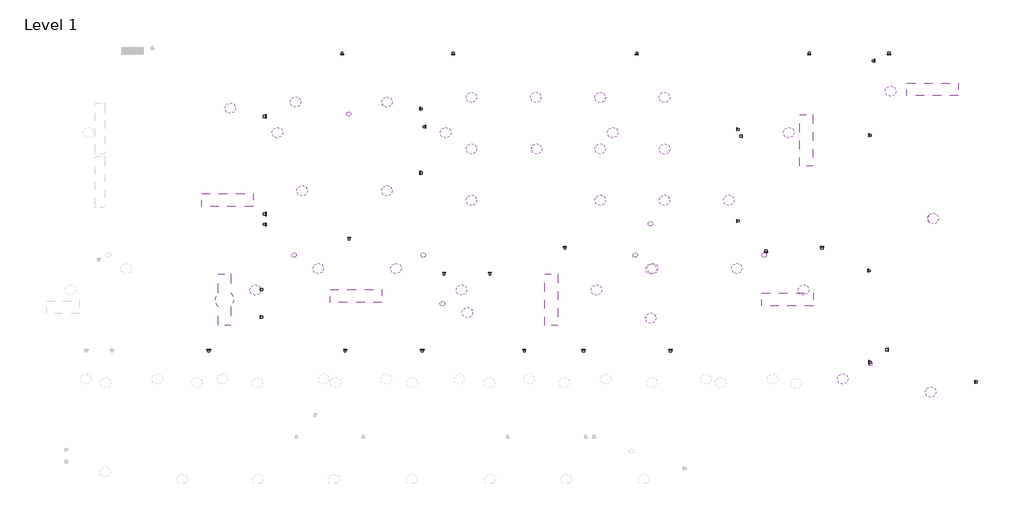
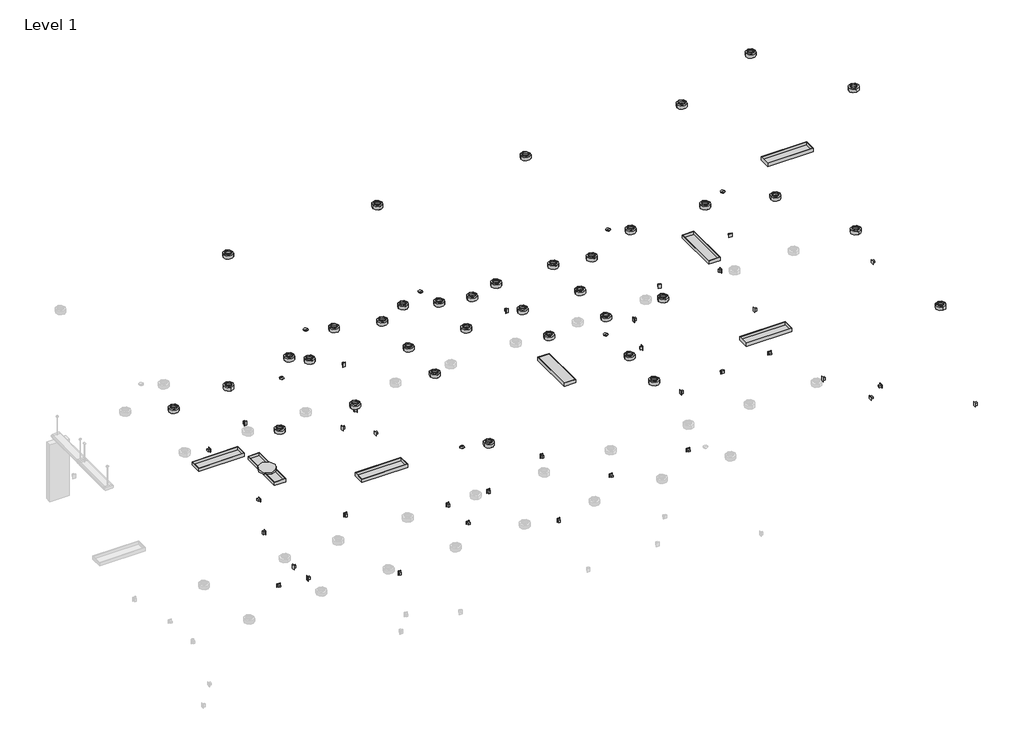
# One storey, part 3 of 3: 43 light fixtures, 22 proxies, 20 switching devices.
# Revit data of these elements (continued)
# Element 74 (IfcSwitchingDevice, "Lighting Switches One Way : One Way Switch") (continued)
#   Mark = "33"
#   COBie.CreatedBy = "info@mma.ie"
#   COBie.CreatedOn = "2017-07-25T10:15:16"
#   COBie.Component.Name = "Lighting Switches One Way_33"
#   COBie.Component.Space = "113"
#   COBie.Component.Description = "Lighting Switches One Way: One Way Switch"
#   Notes = "n/a"
#   Floor Level = "Level 1"
#   COBie = yes
#   Phase Created = New Construction
# Element 75 (IfcSwitchingDevice, "Lighting Switches One Way : One Way Switch")
#   Comments = "Switch"
#   Mark = "34"
#   COBie.CreatedBy = "info@mma.ie"
#   COBie.CreatedOn = "2017-07-25T10:15:16"
#   COBie.Component.Name = "Lighting Switches One Way_34"
#   COBie.Component.Space = "112"
#   COBie.Component.Description = "Lighting Switches One Way: One Way Switch"
#   Notes = "n/a"
#   Floor Level = "Level 1"
#   COBie = yes
#   Phase Created = New Construction
# Element 76 (IfcSwitchingDevice, "Lighting Switches One Way : One Way Switch")
#   Comments = "Switch"
#   Mark = "35"
#   COBie.CreatedBy = "info@mma.ie"
#   COBie.CreatedOn = "2017-07-25T10:15:16"
#   COBie.Component.Name = "Lighting Switches One Way_35"
#   COBie.Component.Space = "111"
#   COBie.Component.Description = "Lighting Switches One Way: One Way Switch"
#   Notes = "n/a"
#   Floor Level = "Level 1"
#   COBie = yes
#   Phase Created = New Construction
# Element 77 (IfcSwitchingDevice, "Lighting Switches One Way : One Way Switch")
#   Comments = "Switch"
#   Mark = "36"
#   COBie.CreatedBy = "info@mma.ie"
#   COBie.CreatedOn = "2017-07-25T10:15:16"
#   COBie.Component.Name = "Lighting Switches One Way_36"
#   COBie.Component.Space = "115"
#   COBie.Component.Description = "Lighting Switches One Way: One Way Switch"
#   Notes = "n/a"
#   Floor Level = "Level 1"
#   COBie = yes
#   Phase Created = New Construction
# Element 78 (IfcSwitchingDevice, "Lighting Switches One Way : One Way Switch")
#   Comments = "Switch"
#   Mark = "37"
#   COBie.CreatedBy = "info@mma.ie"
#   COBie.CreatedOn = "2017-07-25T10:15:16"
#   COBie.Component.Name = "Lighting Switches One Way_37"
#   COBie.Component.Space = "110"
#   COBie.Component.Description = "Lighting Switches One Way: One Way Switch"
#   Notes = "n/a"
#   Floor Level = "Level 1"
#   COBie = yes
#   Phase Created = New Construction
# Element 79 (IfcSwitchingDevice, "Lighting Switches One Way : One Way Switch")
#   Comments = "Switch"
#   Mark = "38"
#   COBie.CreatedBy = "info@mma.ie"
#   COBie.CreatedOn = "2017-07-25T10:15:16"
#   COBie.Component.Name = "Lighting Switches One Way_38"
#   COBie.Component.Space = "109"
#   COBie.Component.Description = "Lighting Switches One Way: One Way Switch"
#   Notes = "n/a"
#   Floor Level = "Level 1"
#   COBie = yes
#   Phase Created = New Construction
# Element 80 (IfcSwitchingDevice, "Lighting Switches One Way : One Way Switch")
#   Comments = "Switch"
#   Mark = "39"
#   COBie.ExternalIdentifier = ""
#   COBie.CreatedBy = "info@mma.ie"
#   COBie.CreatedOn = "2017-07-25T10:15:16"
#   COBie.Component.Name = "Lighting Switches One Way_39"
#   COBie.Component.Space = "108"
#   COBie.Component.Description = "Lighting Switches One Way: One Way Switch"
#   Notes = "n/a"
#   Floor Level = "Level 1"
#   COBie = yes
#   Phase Created = New Construction
# Element 81 (IfcSwitchingDevice, "Lighting Switches One Way : One Way Switch")
#   Comments = "Switch"
#   Mark = "40"
#   COBie.CreatedBy = "info@mma.ie"
#   COBie.CreatedOn = "2017-07-25T10:15:16"
#   COBie.Component.Name = "Lighting Switches One Way_40"
#   COBie.Component.Space = "108"
#   COBie.Component.Description = "Lighting Switches One Way: One Way Switch"
#   Notes = "n/a"
#   Floor Level = "Level 1"
#   COBie = yes
#   Phase Created = New Construction
# Element 82 (IfcSwitchingDevice, "Lighting Switches One Way : One Way Switch")
#   Comments = "Switch"
#   Mark = "41"
#   COBie.CreatedBy = "info@mma.ie"
#   COBie.CreatedOn = "2017-07-25T10:15:16"
#   COBie.Component.Name = "Lighting Switches One Way_41"
#   COBie.Component.Space = "108"
#   COBie.Component.Description = "Lighting Switches One Way: One Way Switch"
#   Notes = "n/a"
#   Floor Level = "Level 1"
#   COBie = yes
#   Phase Created = New Construction
# Element 83 (IfcSwitchingDevice, "Lighting Switches Two Way : Two Way Switch")
#   Comments = "Switch"
#   Mark = "1"
#   COBie.CreatedBy = "info@mma.ie"
#   COBie.CreatedOn = "2017-07-25T10:15:16"
#   COBie.Component.Name = "Lighting Switches Two Way_1"
#   COBie.Component.Space = "117"
#   COBie.Component.Description = "Lighting Switches Two Way: Two Way Switch"
#   Notes = "n/a"
#   Floor Level = "Level 1"
#   COBie = yes
#   Phase Created = New Construction
# Element 84 (IfcSwitchingDevice, "Lighting Switches Two Way : Two Way Switch")
#   Comments = "Switch"
#   Mark = "4"
#   COBie.CreatedBy = "info@mma.ie"
#   COBie.CreatedOn = "2017-07-25T10:15:16"
#   COBie.Component.Name = "Lighting Switches Two Way_4"
#   COBie.Component.Space = "217"
#   COBie.Component.Description = "Lighting Switches Two Way: Two Way Switch"
#   Notes = "n/a"
#   Floor Level = "Level 2"
#   COBie = yes
#   Phase Created = New Construction
# Element 85 (IfcSwitchingDevice, "Lighting Switches Two Way : Two Way Switch")
#   Comments = "Switch"
#   Mark = "2"
#   COBie.CreatedBy = "info@mma.ie"
#   COBie.CreatedOn = "2017-07-25T10:15:16"
#   COBie.Component.Name = "Lighting Switches Two Way_2"
#   COBie.Component.Space = "116"
#   COBie.Component.Description = "Lighting Switches Two Way: Two Way Switch"
#   Notes = "n/a"
#   Floor Level = "Level 1"
#   COBie = yes
#   Phase Created = New Construction
# Materials
#   "Stainless Steel": class "Metal", colour RGB 120 120 120, transparency 0, Description = "Stainless Steel 18/8", Cost = 0
#   "Phase - Demo": class "System", colour RGB 255 0 0, transparency 0.4
#   "Metal - Paint Finish - Ivory, Glossy": class "Paint", colour RGB 247 247 239, transparency 0, Comments = "Rendering appearance not upgraded "
#   "Glass - White, High Luminance": class "Glass", colour RGB 249 250 249, transparency 0.8
#   "Metal - Paint Finish - Dark Grey, Matt": class "Paint", colour RGB 98 98 98, transparency 0
#   "Phase-Demo": class "Unassigned", colour RGB 0 0 0, transparency 0.4, Cost = 0
#   "Plastic-White-Gloss": class "Plastic", colour RGB 255 255 255, transparency 0, Cost = 0
#   "Metal - Chrome": class "Metal", colour RGB 17 17 17, transparency 0, Comments = "Rendering appearance not upgraded "
# Space at (2185.935, -3546.129) mm, phase "New Construction", upper level "Level 1", upper offset 2000 mm, lower offset 0 mm
#   Number = "128"
#   Name = "External Space Level 1"
#   Classification.Space.Number = "13-25 17"
#   Classification.Space.Description = "External Circulation Spaces"
#   COBie.CreatedBy = "info@mma.ie"
#   COBie.CreatedOn = "2017-07-25T10:15:16"
#   COBie.Space.Name = "128"
#   COBie.Space.Category = "13-25 17 : External Circulation Spaces"
#   COBie.Space.Description = "External Circulation Spaces"
#   Actual Lighting Load per area = 0
#   Actual Power Load per area = 0
#   Sensible Heat Gain per person = 0
#   Specified Lighting Load = 0
#   Specified Power Load = 0
#   Latent Heat Gain per person = 0
#   Total Heat Gain per person = 0
#   Area per Person = 0
#   Number of People = 24.3597 (stored number, unit not read)
#   COBie.Space.UsableHeight = 2000 mm
#   COBie.Space.GrossArea = 695.992 m²
#   COBie.Space.NetArea = 0 m²
#   Lighting Load Units = 0
#   Power Load Units = 0
#   Return Airflow = 0
#   Occupancy Unit = -1
#   Condition Type = 2
#   COBie = yes
#   Construction Type = none
# Space at (25106.449, 9340.039) mm, phase "New Construction", upper level "Level 2", upper offset -200 mm, lower offset 0 mm
#   Number = "111"
#   Name = "Storage"
#   Classification.Space.Number = "13-63 13 11"
#   Classification.Space.Description = "Storage Room"
#   COBie.CreatedBy = "info@mma.ie"
#   COBie.CreatedOn = "2017-07-25T10:15:16"
#   COBie.Space.Name = "111"
#   COBie.Space.Category = "13-63 13 11 : Storage Room"
#   COBie.Space.Description = "Storage"
#   Actual Lighting Load per area = 0
#   Actual Power Load per area = 0
#   Sensible Heat Gain per person = 0
#   Specified Lighting Load = 0
#   Specified Power Load = 0
#   Latent Heat Gain per person = 0
#   Total Heat Gain per person = 0
#   Area per Person = 0
#   Number of People = 9.98655 (stored number, unit not read)
#   COBie.Space.UsableHeight = 3600 mm
#   COBie.Space.GrossArea = 5.21302 m²
#   COBie.Space.NetArea = 0 m²
#   Lighting Load Units = 0
#   Power Load Units = 0
#   Return Airflow = 0
#   Occupancy Unit = -1
#   Condition Type = 2
#   COBie = yes
#   Construction Type = none
# Space at (4303.158, 2552.548) mm, phase "New Construction", upper level "Level 2", upper offset -200 mm, lower offset 0 mm
#   Number = "124"
#   Name = "Closet"
#   Classification.Space.Number = "13-63 13 13"
#   Classification.Space.Description = "Closet"
#   COBie.CreatedBy = "info@mma.ie"
#   COBie.CreatedOn = "2017-07-25T10:15:16"
#   COBie.Space.Name = "124"
#   COBie.Space.Category = "13-63 13 13 : Closet"
#   COBie.Space.Description = "Closet"
#   Actual Lighting Load per area = 0
#   Actual Power Load per area = 0
#   Sensible Heat Gain per person = 0
#   Specified Lighting Load = 0
#   Specified Power Load = 0
#   Latent Heat Gain per person = 0
#   Total Heat Gain per person = 0
#   Area per Person = 0
#   Number of People = 5.16564 (stored number, unit not read)
#   COBie.Space.UsableHeight = 3600 mm
#   COBie.Space.GrossArea = 1.97733 m²
#   COBie.Space.NetArea = 0 m²
#   Lighting Load Units = 0
#   Power Load Units = 0
#   Return Airflow = 0
#   Occupancy Unit = -1
#   Condition Type = 2
#   COBie = yes
#   Construction Type = none
# Space at (-3347.4, 10795.629) mm, phase "New Construction", upper level "Level 2", upper offset 0 mm, lower offset 0 mm
#   Number = "001"
#   Name = "Exercise Terrace"
#   Classification.Space.Number = "13-33 11 15 41"
#   Classification.Space.Description = "Exercise Space"
#   COBie.CreatedBy = "info@mma.ie"
#   COBie.CreatedOn = "2017-07-25T10:15:16"
#   COBie.Space.Name = "001"
#   COBie.Space.Category = "13-33 11 15 41 : Exercise Space"
#   COBie.Space.Description = "Exercise Terrace"
#   Actual Lighting Load per area = 0
#   Actual Power Load per area = 0
#   Sensible Heat Gain per person = 0
#   Specified Lighting Load = 0
#   Specified Power Load = 0
#   Latent Heat Gain per person = 0
#   Total Heat Gain per person = 0
#   Area per Person = 0
#   Number of People = 1.64607 (stored number, unit not read)
#   COBie.Space.UsableHeight = 3800 mm
#   COBie.Space.GrossArea = 47.0306 m²
#   COBie.Space.NetArea = 0 m²
#   Lighting Load Units = 0
#   Power Load Units = 0
#   Return Airflow = 0
#   Occupancy Unit = -1
#   Condition Type = 2
#   COBie = yes
#   Construction Type = none
# Space at (19013.47, -3392.114) mm, phase "New Construction", upper level "Level 2", upper offset 0 mm, lower offset 0 mm
#   Number = "002"
#   Name = "Terrace"
#   Classification.Space.Number = "13-33 15 19"
#   Classification.Space.Description = "Recreational Deck"
#   COBie.CreatedBy = "info@mma.ie"
#   COBie.CreatedOn = "2017-07-25T10:15:16"
#   COBie.Space.Name = "002"
#   COBie.Space.Category = "13-33 15 19 : Recreational Deck"
#   COBie.Space.Description = "Terrace"
#   Actual Lighting Load per area = 0
#   Actual Power Load per area = 0
#   Sensible Heat Gain per person = 0
#   Specified Lighting Load = 0
#   Specified Power Load = 0
#   Latent Heat Gain per person = 0
#   Total Heat Gain per person = 0
#   Area per Person = 0
#   Number of People = 4.71044 (stored number, unit not read)
#   COBie.Space.UsableHeight = 3800 mm
#   COBie.Space.GrossArea = 134.584 m²
#   COBie.Space.NetArea = 0 m²
#   Lighting Load Units = 0
#   Power Load Units = 0
#   Return Airflow = 0
#   Occupancy Unit = -1
#   Condition Type = 2
#   COBie = yes
#   Construction Type = none
# Space at (33637.505, 9582.548) mm, phase "New Construction", upper level "Level 2", upper offset 0 mm, lower offset 0 mm
#   Number = "116"
#   Name = "Stair 2"
#   Classification.Space.Number = "13-23 11 13"
#   Classification.Space.Description = "Stairway"
#   COBie.CreatedBy = "info@mma.ie"
#   COBie.CreatedOn = "2017-07-25T10:15:16"
#   COBie.Space.Name = "116"
#   COBie.Space.Category = "13-23 11 13 : Stairway"
#   COBie.Space.Description = "Stair 2"
#   Actual Lighting Load per area = 0
#   Actual Power Load per area = 0
#   Sensible Heat Gain per person = 0
#   Specified Lighting Load = 0
#   Specified Power Load = 0
#   Latent Heat Gain per person = 0
#   Total Heat Gain per person = 0
#   Area per Person = 0
#   Number of People = 0.462 (stored number, unit not read)
#   COBie.Space.UsableHeight = 3800 mm
#   COBie.Space.GrossArea = 11.862 m²
#   COBie.Space.NetArea = 0 m²
#   Lighting Load Units = 0
#   Power Load Units = 0
#   Return Airflow = 0
#   Occupancy Unit = -1
#   Condition Type = 2
#   COBie = yes
#   Construction Type = none
# Space at (13307.53, 9198.989) mm, phase "New Construction", upper level "Level 2", upper offset -200 mm, lower offset 0 mm
#   Number = "104"
#   Name = "Storage"
#   Classification.Space.Number = "13-63 13 11"
#   Classification.Space.Description = "Storage Room"
#   COBie.CreatedBy = "info@mma.ie"
#   COBie.CreatedOn = "2017-07-25T10:15:16"
#   COBie.Space.Name = "104"
#   COBie.Space.Category = "13-63 13 11 : Storage Room"
#   COBie.Space.Description = "Storage"
#   Actual Lighting Load per area = 0
#   Actual Power Load per area = 0
#   Sensible Heat Gain per person = 0
#   Specified Lighting Load = 0
#   Specified Power Load = 0
#   Latent Heat Gain per person = 0
#   Total Heat Gain per person = 0
#   Area per Person = 0
#   Number of People = 0.36309 (stored number, unit not read)
#   COBie.Space.UsableHeight = 3600 mm
#   COBie.Space.GrossArea = 10.374 m²
#   COBie.Space.NetArea = 0 m²
#   Lighting Load Units = 0
#   Power Load Units = 0
#   Return Airflow = 0
#   Occupancy Unit = -1
#   Condition Type = 2
#   COBie = yes
#   Construction Type = none
# Space at (17223.661, 11648.121) mm, phase "New Construction", upper level "Level 2", upper offset -200 mm, lower offset 0 mm
#   Number = "107"
#   Name = "Closet"
#   Classification.Space.Number = "13-63 13 13"
#   Classification.Space.Description = "Closet"
#   COBie.CreatedBy = "info@mma.ie"
#   COBie.CreatedOn = "2017-07-25T10:15:16"
#   COBie.Space.Name = "107"
#   COBie.Space.Category = "13-63 13 13 : Closet"
#   COBie.Space.Description = "Closet"
#   Actual Lighting Load per area = 0
#   Actual Power Load per area = 0
#   Sensible Heat Gain per person = 0
#   Specified Lighting Load = 0
#   Specified Power Load = 0
#   Latent Heat Gain per person = 0
#   Total Heat Gain per person = 0
#   Area per Person = 0
#   Number of People = 0.0932222 (stored number, unit not read)
#   COBie.Space.UsableHeight = 3600 mm
#   COBie.Space.GrossArea = 2.66349 m²
#   COBie.Space.NetArea = 0 m²
#   Lighting Load Units = 0
#   Power Load Units = 0
#   Return Airflow = 0
#   Occupancy Unit = -1
#   Condition Type = 2
#   COBie = yes
#   Construction Type = none
# Space at (17223.661, 9449.227) mm, phase "New Construction", upper level "Level 2", upper offset -200 mm, lower offset 0 mm
#   Number = "109"
#   Name = "Elec/Tel"
#   Classification.Space.Number = "13-23 19 27"
#   Classification.Space.Description = "Electrical Room"
#   COBie.CreatedBy = "info@mma.ie"
#   COBie.CreatedOn = "2017-07-25T10:15:16"
#   COBie.Space.Name = "109"
#   COBie.Space.Category = "13-23 19 27 : Electrical Room"
#   COBie.Space.Description = "Elec/Tel"
#   Actual Lighting Load per area = 0
#   Actual Power Load per area = 0
#   Sensible Heat Gain per person = 0
#   Specified Lighting Load = 0
#   Specified Power Load = 0
#   Latent Heat Gain per person = 0
#   Total Heat Gain per person = 0
#   Area per Person = 0
#   Number of People = 0.141204 (stored number, unit not read)
#   COBie.Space.UsableHeight = 3600 mm
#   COBie.Space.GrossArea = 4.03441 m²
#   COBie.Space.NetArea = 0 m²
#   Lighting Load Units = 0
#   Power Load Units = 0
#   Return Airflow = 0
#   Occupancy Unit = -1
#   Condition Type = 2
#   COBie = yes
#   Construction Type = none
# Space at (20994.03, 9449.227) mm, phase "New Construction", upper level "Level 2", upper offset -200 mm, lower offset 0 mm
#   Number = "110"
#   Name = "Laundry"
#   Classification.Space.Number = "13-65 17"
#   Classification.Space.Description = "Laundry Room"
#   COBie.CreatedBy = "info@mma.ie"
#   COBie.CreatedOn = "2017-07-25T10:15:16"
#   COBie.Space.Name = "110"
#   COBie.Space.Category = "13-65 17 : Laundry Room"
#   COBie.Space.Description = "Laundry"
#   Actual Lighting Load per area = 0
#   Actual Power Load per area = 0
#   Sensible Heat Gain per person = 0
#   Specified Lighting Load = 0
#   Specified Power Load = 0
#   Latent Heat Gain per person = 0
#   Total Heat Gain per person = 0
#   Area per Person = 0
#   Number of People = 0.437432 (stored number, unit not read)
#   COBie.Space.UsableHeight = 3600 mm
#   COBie.Space.GrossArea = 12.4981 m²
#   COBie.Space.NetArea = 0 m²
#   Lighting Load Units = 0
#   Power Load Units = 0
#   Return Airflow = 0
#   Occupancy Unit = -1
#   Condition Type = 2
#   COBie = yes
#   Construction Type = none
# Space at (9483.268, 9198.989) mm, phase "New Construction", upper level "Level 2", upper offset -200 mm, lower offset 0 mm
#   Number = "103"
#   Name = "Toilet"
#   Classification.Space.Number = "13-65 13 13"
#   Classification.Space.Description = "Toilet Space"
#   COBie.CreatedBy = "info@mma.ie"
#   COBie.CreatedOn = "2017-07-25T10:15:16"
#   COBie.Space.Name = "103"
#   COBie.Space.Category = "13-65 13 13 : Toilet Space"
#   COBie.Space.Description = "Toilet"
#   Actual Lighting Load per area = 0
#   Actual Power Load per area = 0
#   Sensible Heat Gain per person = 0
#   Specified Lighting Load = 0
#   Specified Power Load = 0
#   Latent Heat Gain per person = 0
#   Total Heat Gain per person = 0
#   Area per Person = 0
#   Number of People = 0.146893 (stored number, unit not read)
#   COBie.Space.UsableHeight = 3600 mm
#   COBie.Space.GrossArea = 4.19694 m²
#   COBie.Space.NetArea = 0 m²
#   Lighting Load Units = 0
#   Power Load Units = 0
#   Return Airflow = 0
#   Occupancy Unit = -1
#   Condition Type = 2
#   COBie = yes
#   Construction Type = none
# Space at (7140.705, 9198.989) mm, phase "New Construction", upper level "Level 2", upper offset -200 mm, lower offset 0 mm
#   Number = "102"
#   Name = "Toilet"
#   Classification.Space.Number = "13-65 13 13"
#   Classification.Space.Description = "Toilet Space"
#   COBie.CreatedBy = "info@mma.ie"
#   COBie.CreatedOn = "2017-07-25T10:15:16"
#   COBie.Space.Name = "102"
#   COBie.Space.Category = "13-65 13 13 : Toilet Space"
#   COBie.Space.Description = "Toilet"
#   Actual Lighting Load per area = 0
#   Actual Power Load per area = 0
#   Sensible Heat Gain per person = 0
#   Specified Lighting Load = 0
#   Specified Power Load = 0
#   Latent Heat Gain per person = 0
#   Total Heat Gain per person = 0
#   Area per Person = 0
#   Number of People = 0.146751 (stored number, unit not read)
#   COBie.Space.UsableHeight = 3600 mm
#   COBie.Space.GrossArea = 4.19289 m²
#   COBie.Space.NetArea = 0 m²
#   Lighting Load Units = 0
#   Power Load Units = 0
#   Return Airflow = 0
#   Occupancy Unit = -1
#   Condition Type = 2
#   COBie = yes
#   Construction Type = none
# Space at (17223.661, 13855.183) mm, phase "New Construction", upper level "Level 2", upper offset -200 mm, lower offset 0 mm
#   Number = "106"
#   Name = "Bath"
#   Classification.Space.Number = "13-65 13"
#   Classification.Space.Description = "Bathroom"
#   COBie.CreatedBy = "info@mma.ie"
#   COBie.CreatedOn = "2017-07-25T10:15:16"
#   COBie.Space.Name = "106"
#   COBie.Space.Category = "13-65 13 : Bathroom"
#   COBie.Space.Description = "Bath"
#   Actual Lighting Load per area = 0
#   Actual Power Load per area = 0
#   Sensible Heat Gain per person = 0
#   Specified Lighting Load = 0
#   Specified Power Load = 0
#   Latent Heat Gain per person = 0
#   Total Heat Gain per person = 0
#   Area per Person = 0
#   Number of People = 0.141421 (stored number, unit not read)
#   COBie.Space.UsableHeight = 3600 mm
#   COBie.Space.GrossArea = 4.0406 m²
#   COBie.Space.NetArea = 0 m²
#   Lighting Load Units = 0
#   Power Load Units = 0
#   Return Airflow = 0
#   Occupancy Unit = -1
#   Condition Type = 2
#   COBie = yes
#   Construction Type = none
# Space at (19950.249, 12967.977) mm, phase "New Construction", upper level "Level 2", upper offset -200 mm, lower offset 0 mm
#   Number = "108"
#   Name = "Break Room"
#   Classification.Space.Number = "13-57 17 13"
#   Classification.Space.Description = "Break Room"
#   COBie.CreatedBy = "info@mma.ie"
#   COBie.CreatedOn = "2017-07-25T10:15:16"
#   COBie.Space.Name = "108"
#   COBie.Space.Category = "13-57 17 13 : Break Room"
#   COBie.Space.Description = "Break Room"
#   Actual Lighting Load per area = 0
#   Actual Power Load per area = 0
#   Sensible Heat Gain per person = 0
#   Specified Lighting Load = 0
#   Specified Power Load = 0
#   Latent Heat Gain per person = 0
#   Total Heat Gain per person = 0
#   Area per Person = 0
#   Number of People = 0.538984 (stored number, unit not read)
#   COBie.Space.UsableHeight = 3600 mm
#   COBie.Space.GrossArea = 15.3995 m²
#   COBie.Space.NetArea = 0 m²
#   Lighting Load Units = 0
#   Power Load Units = 0
#   Return Airflow = 0
#   Occupancy Unit = -1
#   Condition Type = 2
#   COBie = yes
#   Construction Type = none
# Space at (33531.255, 14017.548) mm, phase "New Construction", upper level "Level 2", upper offset -200 mm, lower offset 0 mm
#   Number = "115"
#   Name = "Outdoor Storage"
#   Classification.Space.Number = "13-63 13 11"
#   Classification.Space.Description = "Storage Room"
#   COBie.CreatedBy = "info@mma.ie"
#   COBie.CreatedOn = "2017-07-25T10:15:16"
#   COBie.Space.Name = "115"
#   COBie.Space.Category = "13-63 13 11 : Storage Room"
#   COBie.Space.Description = "Outdoor Storage"
#   Actual Lighting Load per area = 0
#   Actual Power Load per area = 0
#   Sensible Heat Gain per person = 0
#   Specified Lighting Load = 0
#   Specified Power Load = 0
#   Latent Heat Gain per person = 0
#   Total Heat Gain per person = 0
#   Area per Person = 0
#   Number of People = 0.183416 (stored number, unit not read)
#   COBie.Space.UsableHeight = 3600 mm
#   COBie.Space.GrossArea = 5.24046 m²
#   COBie.Space.NetArea = 0 m²
#   Lighting Load Units = 0
#   Power Load Units = 0
#   Return Airflow = 0
#   Occupancy Unit = -1
#   Condition Type = 2
#   COBie = yes
#   Construction Type = none
# Space at (12208.83, 12750.239) mm, phase "New Construction", upper level "Level 2", upper offset -200 mm, lower offset 0 mm
#   Number = "105"
#   Name = "Mechanical Room"
#   Classification.Space.Number = "13-23 19"
#   Classification.Space.Description = "Utility Equipment Room"
#   COBie.CreatedBy = "info@mma.ie"
#   COBie.CreatedOn = "2017-07-25T10:15:16"
#   COBie.Space.Name = "105"
#   COBie.Space.Category = "13-23 19 : Utility Equipment Room"
#   COBie.Space.Description = "Mechanical Room"
#   Actual Lighting Load per area = 0
#   Actual Power Load per area = 0
#   Sensible Heat Gain per person = 0
#   Specified Lighting Load = 0
#   Specified Power Load = 0
#   Latent Heat Gain per person = 0
#   Total Heat Gain per person = 0
#   Area per Person = 0
#   Number of People = 1.28766 (stored number, unit not read)
#   COBie.Space.UsableHeight = 3600 mm
#   COBie.Space.GrossArea = 36.7902 m²
#   COBie.Space.NetArea = 0 m²
#   Lighting Load Units = 0
#   Power Load Units = 0
#   Return Airflow = 0
#   Occupancy Unit = -1
#   Condition Type = 2
#   COBie = yes
#   Construction Type = none
# Space at (10643.485, 2189.772) mm, phase "New Construction", upper level "Level 2", upper offset -200 mm, lower offset 0 mm
#   Number = "121"
#   Name = "Living Room"
#   Classification.Space.Number = "13-65"
#   Classification.Space.Description = "Private Residential Spaces"
#   COBie.CreatedBy = "info@mma.ie"
#   COBie.CreatedOn = "2017-07-25T10:15:16"
#   COBie.Space.Name = "121"
#   COBie.Space.Category = "13-57 17 11 : Rest Area"
#   COBie.Space.Description = "Living Room"
#   Actual Lighting Load per area = 0
#   Actual Power Load per area = 0
#   Sensible Heat Gain per person = 0
#   Specified Lighting Load = 0
#   Specified Power Load = 0
#   Latent Heat Gain per person = 0
#   Total Heat Gain per person = 0
#   Area per Person = 0
#   Number of People = 0.615682 (stored number, unit not read)
#   COBie.Space.UsableHeight = 3600 mm
#   COBie.Space.GrossArea = 17.5909 m²
#   COBie.Space.NetArea = 0 m²
#   Lighting Load Units = 0
#   Power Load Units = 0
#   Return Airflow = 0
#   Occupancy Unit = -1
#   Condition Type = 2
#   COBie = yes
#   Construction Type = none
# Space at (9068.854, 5264.772) mm, phase "New Construction", upper level "Level 2", upper offset -200 mm, lower offset 0 mm
#   Number = "122"
#   Name = "Closet"
#   Classification.Space.Number = "13-63 13 13"
#   Classification.Space.Description = "Closet"
#   COBie.CreatedBy = "info@mma.ie"
#   COBie.CreatedOn = "2017-07-25T10:15:16"
#   COBie.Space.Name = "122"
#   COBie.Space.Category = "13-63 13 13 : Closet"
#   COBie.Space.Description = "Closet"
#   Actual Lighting Load per area = 0
#   Actual Power Load per area = 0
#   Sensible Heat Gain per person = 0
#   Specified Lighting Load = 0
#   Specified Power Load = 0
#   Latent Heat Gain per person = 0
#   Total Heat Gain per person = 0
#   Area per Person = 0
#   Number of People = 0.113917 (stored number, unit not read)
#   COBie.Space.UsableHeight = 3600 mm
#   COBie.Space.GrossArea = 3.25478 m²
#   COBie.Space.NetArea = 0 m²
#   Lighting Load Units = 0
#   Power Load Units = 0
#   Return Airflow = 0
#   Occupancy Unit = -1
#   Condition Type = 2
#   COBie = yes
#   Construction Type = none
# Space at (3785.935, 3859.219) mm, phase "New Construction", upper level "Level 2", upper offset 0 mm, lower offset 0 mm
#   Number = "125"
#   Name = "Stair 1"
#   Classification.Space.Number = "13-23 11 13"
#   Classification.Space.Description = "Stairway"
#   COBie.CreatedBy = "info@mma.ie"
#   COBie.CreatedOn = "2017-07-25T10:15:16"
#   COBie.Space.Name = "125"
#   COBie.Space.Category = "13-23 11 13 : Stairway"
#   COBie.Space.Description = "Stair 1"
#   Actual Lighting Load per area = 0
#   Actual Power Load per area = 0
#   Sensible Heat Gain per person = 0
#   Specified Lighting Load = 0
#   Specified Power Load = 0
#   Latent Heat Gain per person = 0
#   Total Heat Gain per person = 0
#   Area per Person = 0
#   Number of People = 0.341177 (stored number, unit not read)
#   COBie.Space.UsableHeight = 3800 mm
#   COBie.Space.GrossArea = 9.74791 m²
#   COBie.Space.NetArea = 0 m²
#   Lighting Load Units = 0
#   Power Load Units = 0
#   Return Airflow = 0
#   Occupancy Unit = -1
#   Condition Type = 2
#   COBie = yes
#   Construction Type = none
# Space at (25507.293, 11656.289) mm, phase "New Construction", upper level "Level 2", upper offset -200 mm, lower offset 0 mm
#   Number = "112"
#   Name = "Kitchen"
#   Classification.Space.Number = "13-57 13 13"
#   Classification.Space.Description = "Kitchen Space"
#   COBie.CreatedBy = "info@mma.ie"
#   COBie.CreatedOn = "2017-07-25T10:15:16"
#   COBie.Space.Name = "112"
#   COBie.Space.Category = "13-57 13 13 : Kitchen Space"
#   COBie.Space.Description = "Kitchen"
#   Actual Lighting Load per area = 0
#   Actual Power Load per area = 0
#   Sensible Heat Gain per person = 0
#   Specified Lighting Load = 0
#   Specified Power Load = 0
#   Latent Heat Gain per person = 0
#   Total Heat Gain per person = 0
#   Area per Person = 0
#   Number of People = 1.29962 (stored number, unit not read)
#   COBie.Space.UsableHeight = 3600 mm
#   COBie.Space.GrossArea = 37.132 m²
#   COBie.Space.NetArea = 0 m²
#   Lighting Load Units = 0
#   Power Load Units = 0
#   Return Airflow = 0
#   Occupancy Unit = -1
#   Condition Type = 2
#   COBie = yes
#   Construction Type = none
# Space at (11800.436, 5264.772) mm, phase "New Construction", upper level "Level 2", upper offset -200 mm, lower offset 0 mm
#   Number = "120"
#   Name = "Storage"
#   Classification.Space.Number = "13-63 13 11"
#   Classification.Space.Description = "Storage Room"
#   COBie.CreatedBy = "info@mma.ie"
#   COBie.CreatedOn = "2017-07-25T10:15:16"
#   COBie.Space.Name = "120"
#   COBie.Space.Category = "13-63 13 11 : Storage Room"
#   COBie.Space.Description = "Storage"
#   Actual Lighting Load per area = 0
#   Actual Power Load per area = 0
#   Sensible Heat Gain per person = 0
#   Specified Lighting Load = 0
#   Specified Power Load = 0
#   Latent Heat Gain per person = 0
#   Total Heat Gain per person = 0
#   Area per Person = 0
#   Number of People = 0.214926 (stored number, unit not read)
#   COBie.Space.UsableHeight = 3600 mm
#   COBie.Space.GrossArea = 6.14073 m²
#   COBie.Space.NetArea = 0 m²
#   Lighting Load Units = 0
#   Power Load Units = 0
#   Return Airflow = 0
#   Occupancy Unit = -1
#   Condition Type = 2
#   COBie = yes
#   Construction Type = none
# Space at (14024.524, 3150.039) mm, phase "New Construction", upper level "Level 2", upper offset -200 mm, lower offset 0 mm
#   Number = "119"
#   Name = "Bar"
#   Classification.Space.Number = "13-57 13 15"
#   Classification.Space.Description = "ining and Drinking Spaces"
#   COBie.CreatedBy = "info@mma.ie"
#   COBie.CreatedOn = "2017-07-25T10:15:16"
#   COBie.Space.Name = "119"
#   COBie.Space.Category = "13-57 13 15 : Dining and Drinking Spaces"
#   COBie.Space.Description = "Bar"
#   Actual Lighting Load per area = 0
#   Actual Power Load per area = 0
#   Sensible Heat Gain per person = 0
#   Specified Lighting Load = 0
#   Specified Power Load = 0
#   Latent Heat Gain per person = 0
#   Total Heat Gain per person = 0
#   Area per Person = 0
#   Number of People = 0.412197 (stored number, unit not read)
#   COBie.Space.UsableHeight = 3600 mm
#   COBie.Space.GrossArea = 11.7771 m²
#   COBie.Space.NetArea = 0 m²
#   Lighting Load Units = 0
#   Power Load Units = 0
#   Return Airflow = 0
#   Occupancy Unit = -1
#   Condition Type = 2
#   COBie = yes
#   Construction Type = none
# Space at (30744.455, 12858.789) mm, phase "New Construction", upper level "Level 2", upper offset -200 mm, lower offset 0 mm
#   Number = "113"
#   Name = "Food Storage"
#   Classification.Space.Number = "13-63 13 11"
#   Classification.Space.Description = "Storage Room"
#   COBie.CreatedBy = "info@mma.ie"
#   COBie.CreatedOn = "2017-07-25T10:15:16"
#   COBie.Space.Name = "113"
#   COBie.Space.Category = "13-63 13 11 : Storage Room"
#   COBie.Space.Description = "Food Storage"
#   Actual Lighting Load per area = 0
#   Actual Power Load per area = 0
#   Sensible Heat Gain per person = 0
#   Specified Lighting Load = 0
#   Specified Power Load = 0
#   Latent Heat Gain per person = 0
#   Total Heat Gain per person = 0
#   Area per Person = 0
#   Number of People = 0.465855 (stored number, unit not read)
#   COBie.Space.UsableHeight = 3600 mm
#   COBie.Space.GrossArea = 13.3101 m²
#   COBie.Space.NetArea = 0 m²
#   Lighting Load Units = 0
#   Power Load Units = 0
#   Return Airflow = 0
#   Occupancy Unit = -1
#   Condition Type = 2
#   COBie = yes
#   Construction Type = none
# Space at (30095.168, 9340.039) mm, phase "New Construction", upper level "Level 2", upper offset -200 mm, lower offset 0 mm
#   Number = "114"
#   Name = "Pantry"
#   Classification.Space.Number = "13-57 13 13"
#   Classification.Space.Description = "Kitchen Space"
#   COBie.CreatedBy = "info@mma.ie"
#   COBie.CreatedOn = "2017-07-25T10:15:16"
#   COBie.Space.Name = "114"
#   COBie.Space.Category = "13-57 13 13 : Kitchen Space"
#   COBie.Space.Description = "Pantry"
#   Actual Lighting Load per area = 0
#   Actual Power Load per area = 0
#   Sensible Heat Gain per person = 0
#   Specified Lighting Load = 0
#   Specified Power Load = 0
#   Latent Heat Gain per person = 0
#   Total Heat Gain per person = 0
#   Area per Person = 0
#   Number of People = 0.339922 (stored number, unit not read)
#   COBie.Space.UsableHeight = 3600 mm
#   COBie.Space.GrossArea = 9.71206 m²
#   COBie.Space.NetArea = 0 m²
#   Lighting Load Units = 0
#   Power Load Units = 0
#   Return Airflow = 0
#   Occupancy Unit = -1
#   Condition Type = 2
#   COBie = yes
#   Construction Type = none
# Space at (4246.33, 10900.039) mm, phase "New Construction", upper level "Level 2", upper offset -200 mm, lower offset 0 mm
#   Number = "101"
#   Name = "Exercise Room"
#   Classification.Space.Number = "13-33 11 15 41"
#   Classification.Space.Description = "Exercise Space"
#   COBie.CreatedBy = "info@mma.ie"
#   COBie.CreatedOn = "2017-07-25T10:15:16"
#   COBie.Space.Name = "101"
#   COBie.Space.Category = "13-33 11 15 41 : Exercise Space"
#   COBie.Space.Description = "Exercise Room"
#   Actual Lighting Load per area = 0
#   Actual Power Load per area = 0
#   Sensible Heat Gain per person = 0
#   Specified Lighting Load = 0
#   Specified Power Load = 0
#   Latent Heat Gain per person = 0
#   Total Heat Gain per person = 0
#   Area per Person = 0
#   Number of People = 2.09985 (stored number, unit not read)
#   COBie.Space.UsableHeight = 3600 mm
#   COBie.Space.GrossArea = 59.9957 m²
#   COBie.Space.NetArea = 0 m²
#   Lighting Load Units = 0
#   Power Load Units = 0
#   Return Airflow = 0
#   Occupancy Unit = -1
#   Condition Type = 2
#   COBie = yes
#   Construction Type = none
# Space at (19128.717, 7268.789) mm, phase "New Construction", upper level "Level 2", upper offset -200 mm, lower offset 0 mm
#   Number = "117"
#   Name = "Hall"
#   Classification.Space.Number = "13-25"
#   Classification.Space.Description = "Circulation Spaces"
#   COBie.CreatedBy = "info@mma.ie"
#   COBie.CreatedOn = "2017-07-25T10:15:16"
#   COBie.Space.Name = "117"
#   COBie.Space.Category = "13-25 : Circulation Spaces"
#   COBie.Space.Description = "Hall"
#   Actual Lighting Load per area = 0
#   Actual Power Load per area = 0
#   Sensible Heat Gain per person = 0
#   Specified Lighting Load = 0
#   Specified Power Load = 0
#   Latent Heat Gain per person = 0
#   Total Heat Gain per person = 0
#   Area per Person = 0
#   Number of People = 1.29126 (stored number, unit not read)
#   COBie.Space.UsableHeight = 3600 mm
#   COBie.Space.GrossArea = 36.893 m²
#   COBie.Space.NetArea = 0 m²
#   Lighting Load Units = 0
#   Power Load Units = 0
#   Return Airflow = 0
#   Occupancy Unit = -1
#   Condition Type = 2
#   COBie = yes
#   Construction Type = none
# Space at (6812.839, 4751.96) mm, phase "New Construction", upper level "Level 2", upper offset -200 mm, lower offset 0 mm
#   Number = "123"
#   Name = "Entry"
#   Classification.Space.Number = "13-25"
#   Classification.Space.Description = "Circulation Spaces"
#   COBie.CreatedBy = "info@mma.ie"
#   COBie.CreatedOn = "2017-07-25T10:15:16"
#   COBie.Space.Name = "123"
#   COBie.Space.Category = "13-25 : Circulation Spaces"
#   COBie.Space.Description = "Entry"
#   Actual Lighting Load per area = 0
#   Actual Power Load per area = 0
#   Sensible Heat Gain per person = 0
#   Specified Lighting Load = 0
#   Specified Power Load = 0
#   Latent Heat Gain per person = 0
#   Total Heat Gain per person = 0
#   Area per Person = 0
#   Number of People = 0.264502 (stored number, unit not read)
#   COBie.Space.UsableHeight = 3600 mm
#   COBie.Space.GrossArea = 7.55719 m²
#   COBie.Space.NetArea = 0 m²
#   Lighting Load Units = 0
#   Power Load Units = 0
#   Return Airflow = 0
#   Occupancy Unit = -1
#   Condition Type = 2
#   COBie = yes
#   Construction Type = none
# Space at (21024.121, 3251.566) mm, phase "New Construction", upper level "Level 2", upper offset -200 mm, lower offset 0 mm
#   Number = "118"
#   Name = "Recreation/Dining Room"
#   Classification.Space.Number = "13-57 13 15"
#   Classification.Space.Description = "Dining and Drinking Spaces"
#   COBie.CreatedBy = "info@mma.ie"
#   COBie.CreatedOn = "2017-07-25T10:15:16"
#   COBie.Space.Name = "118"
#   COBie.Space.Category = "13-57 13 15 : Dining and Drinking Spaces"
#   COBie.Space.Description = "Recreation/Dining Room"
#   Actual Lighting Load per area = 0
#   Actual Power Load per area = 0
#   Sensible Heat Gain per person = 0
#   Specified Lighting Load = 0
#   Specified Power Load = 0
#   Latent Heat Gain per person = 0
#   Total Heat Gain per person = 0
#   Area per Person = 0
#   Number of People = 2.68308 (stored number, unit not read)
#   COBie.Space.UsableHeight = 3600 mm
#   COBie.Space.GrossArea = 76.6595 m²
#   COBie.Space.NetArea = 0 m²
#   Lighting Load Units = 0
#   Power Load Units = 0
#   Return Airflow = 0
#   Occupancy Unit = -1
#   Condition Type = 2
#   COBie = yes
#   Construction Type = none
